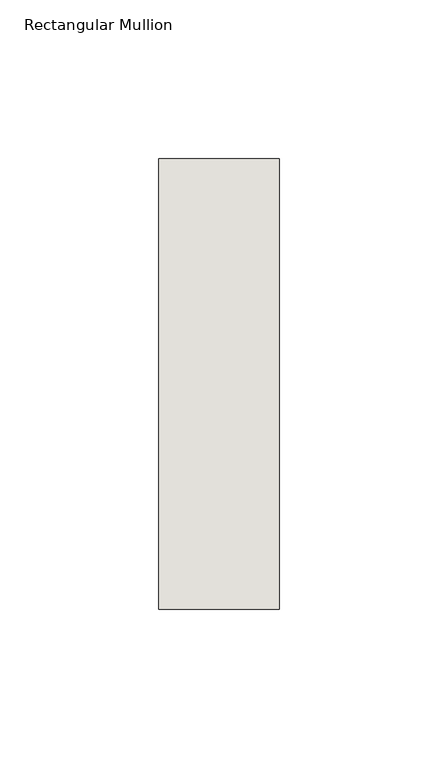
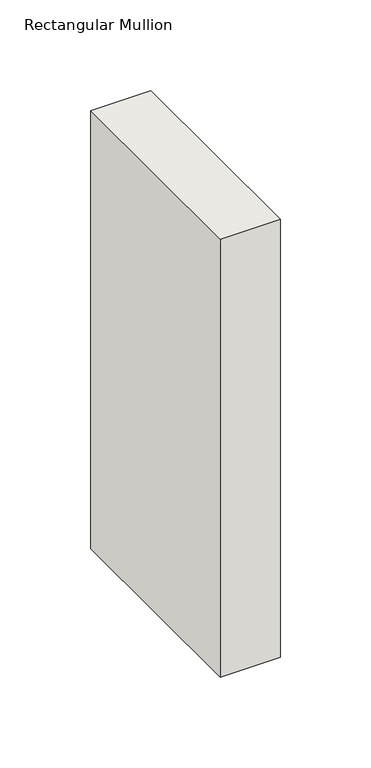
"""IFC4 building model written with IfcOpenShell, lengths in millimetres: wall geometry, Rectangular Mullion : NLRS_21_CWM_hsb-regel 38x142_gen_rsf."""

from ifc_helpers import new_model, si_unit, frame, origin, place, context, project, spatial, polyline, outline, extrude, source, transform, mapped, element, save


def rectangular_mullion_45838a12(model_context):
    return source(origin(), model_context, "Body", "SweptSolid", [
        extrude(outline(polyline([(19.0, -71.0), (-19.0, -71.0), (-19.0, 71.0), (19.0, 71.0), (19.0, -71.0)])), frame((0.0, 0.0, -293.8441061), z_axis=(0.0, 0.0, 1.0), x_axis=(1.0, 0.0, 0.0)), (0.0, 0.0, 1.0), 293.8441061),
    ])


if __name__ == "__main__":
    model = new_model("IFC4")
    model_context = context("Model", 3, world=origin())
    ifc_project = project(units=[si_unit("LENGTHUNIT", "METRE", prefix="MILLI")], contexts=[model_context])
    site = spatial("IfcSite", under=ifc_project)
    building = spatial("IfcBuilding", under=site)
    placement = place(None, origin())
    rectangular_mullion_shape = rectangular_mullion_45838a12(model_context)
    element("IfcWall", 1, ObjectType="Rectangular Mullion : NLRS_21_CWM_hsb-regel 38x142_gen_rsf", at=placement, inside=building, context=model_context, shape_type="MappedRepresentation", body=[
        mapped(rectangular_mullion_shape, transform((0.0, 0.0, 0.0), x_axis=(1.0, 0.0, 0.0), y_axis=(0.0, 1.0, 0.0), z_axis=(0.0, 0.0, 1.0))),
    ])
    save(model, "model.ifc")

# Revit data of these elements
# Type "Rectangular Mullion : NLRS_21_CWM_hsb-regel 38x142_gen_rsf"
#   Type IfcGUID = "07M7mRoiH1CR8m_RSKIwpF"
#   Assembly Code = "21.10"
#   IfcExportAs = "IfcWall"
#   built-in parameter 1007322 = 0.465879 (stored number, unit not read)
#   built-in parameter 1007321 = 0.062336 (stored number, unit not read)
#   built-in parameter 1007320 = 0.062336 (stored number, unit not read)
# Element 1 (IfcWall, "Rectangular Mullion : NLRS_21_CWM_hsb-regel 38x142_gen_rsf")
#   Materials on its faces: "NLRS_i2_hout naaldhout vuren_gen_rsf"
# Materials
#   "NLRS_i2_hout naaldhout vuren_gen_rsf": class "I - Hout", colour RGB 234 199 147, transparency 0, Keynote = "i2", Manufacturer = "Revit Standards Foundation", URL = "www.revitstandards.org", Description = "hout vuren", Cost = 0
